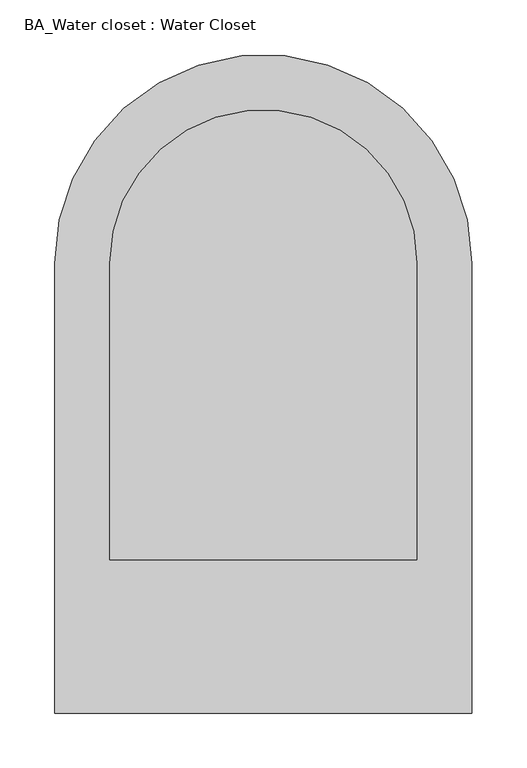
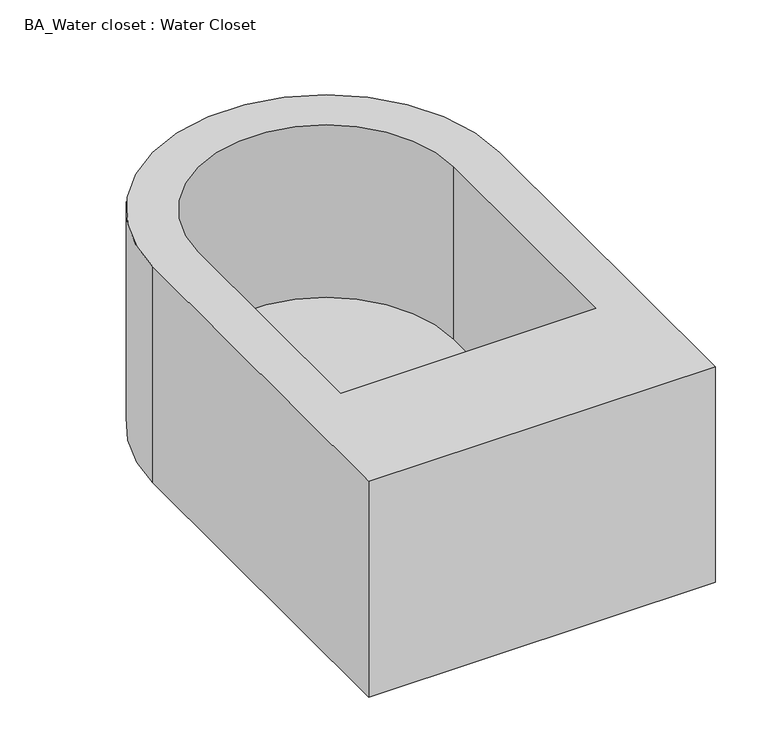
"""IFC4 building model written with IfcOpenShell, lengths in millimetres: flow terminal geometry, BA_Water closet : Water Closet."""

from ifc_helpers import new_model, si_unit, frame, origin, place, context, project, spatial, polyline, circle_curve, source, transform, mapped, element, save
from ifc_brep_helpers import plane_surface, cylinder_surface, revolved_surface, advanced_brep


def ba_water_closet_water_closet_d6486678(model_context):
    return source(origin(), model_context, "Body", "AdvancedBrep", [
        advanced_brep(
        [(-65.0, 560.0, 400.0), (-65.0, 150.0, 400.0), (315.0, 150.0, 400.0), (315.0, 560.0, 400.0), (-15.0, 290.0, 400.0), (-15.0, 560.0, 400.0), (265.0, 560.0, 400.0), (265.0, 290.0, 400.0), (-65.0, 560.0, 150.0), (315.0, 560.0, 150.0), (315.0, 150.0, 150.0), (-65.0, 150.0, 150.0), (-15.0, 560.0, 200.0), (-15.0, 290.0, 200.0), (265.0, 290.0, 200.0), (265.0, 560.0, 200.0)],
        [
            (0, 1),
            (1, 2),
            (2, 3),
            (3, 0, circle_curve(frame((125.0, 560.0, 400.0), z_axis=(0.0, 0.0, 1.0), x_axis=(-1.0, 0.0, 0.0)), 190.0)),
            (4, 5),
            (5, 6, circle_curve(frame((125.0, 560.0, 400.0), z_axis=(0.0, 0.0, -1.0), x_axis=(-1.0, 0.0, 0.0)), 140.0)),
            (6, 7),
            (7, 4),
            (8, 9, circle_curve(frame((125.0, 560.0, 150.0), z_axis=(0.0, 0.0, -1.0), x_axis=(-1.0, 0.0, 0.0)), 190.0)),
            (9, 10),
            (10, 11),
            (11, 8),
            (0, 8),
            (11, 1),
            (10, 2),
            (9, 3),
            (12, 13),
            (13, 14),
            (14, 15),
            (15, 12, circle_curve(frame((125.0, 560.0, 200.0), z_axis=(0.0, 0.0, 1.0), x_axis=(-1.0, 0.0, 0.0)), 140.0)),
            (12, 5),
            (4, 13),
            (7, 14),
            (6, 15),
        ],
        [
            plane_surface(frame((-65.0, 150.0, 400.0), z_axis=(0.0, 0.0, 1.0), x_axis=(0.0, -1.0, 0.0))),
            plane_surface(frame((-65.0, 150.0, 150.0), z_axis=(0.0, 0.0, -1.0), x_axis=(0.0, 1.0, 0.0))),
            plane_surface(frame((-65.0, 560.0, 400.0), z_axis=(-1.0, 0.0, 0.0), x_axis=(0.0, 0.0, -1.0))),
            plane_surface(frame((-65.0, 150.0, 400.0), z_axis=(0.0, -1.0, 0.0), x_axis=(0.0, 0.0, -1.0))),
            plane_surface(frame((315.0, 150.0, 400.0), z_axis=(1.0, 0.0, 0.0), x_axis=(0.0, 0.0, -1.0))),
            plane_surface(frame((-15.0, 290.0, 200.0), z_axis=(0.0, 0.0, 1.0), x_axis=(0.0, 1.0, 0.0))),
            plane_surface(frame((-15.0, 560.0, 400.0), z_axis=(1.0, 0.0, 0.0), x_axis=(0.0, 0.0, -1.0))),
            plane_surface(frame((-15.0, 290.0, 400.0), z_axis=(0.0, 1.0, 0.0), x_axis=(0.0, 0.0, -1.0))),
            plane_surface(frame((265.0, 290.0, 400.0), z_axis=(-1.0, 0.0, 0.0), x_axis=(0.0, 0.0, -1.0))),
            cylinder_surface(frame((125.0, 560.0, 150.0), z_axis=(0.0, 0.0, 1.0), x_axis=(-1.0, 0.0, 0.0)), 190.0),
            revolved_surface(polyline([(-15.0, 560.0, 400.0), (-15.0, 560.0, 200.0)]), (125.0, 560.0, 200.0), (0.0, 0.0, 1.0)),
        ],
        [
            (0, [[1, 2, 3, 4], [5, 6, 7, 8]]),
            (1, [[9, 10, 11, 12]]),
            (2, [[-1, 13, -12, 14]]),
            (3, [[-2, -14, -11, 15]]),
            (4, [[-3, -15, -10, 16]]),
            (5, [[17, 18, 19, 20]]),
            (6, [[-17, 21, -5, 22]]),
            (7, [[-18, -22, -8, 23]]),
            (8, [[-19, -23, -7, 24]]),
            (9, [[-4, -16, -9, -13]]),
            (10, [[-20, -24, -6, -21]]),
        ],
    ),
    ])


if __name__ == "__main__":
    model = new_model("IFC4")
    model_context = context("Model", 3, world=origin())
    ifc_project = project(units=[si_unit("LENGTHUNIT", "METRE", prefix="MILLI")], contexts=[model_context])
    site = spatial("IfcSite", under=ifc_project)
    building = spatial("IfcBuilding", under=site)
    placement = place(None, origin())
    ba_water_closet_water_closet_shape = ba_water_closet_water_closet_d6486678(model_context)
    element("IfcFlowTerminal", 1, ObjectType="BA_Water closet : Water Closet", at=placement, inside=building, context=model_context, shape_type="MappedRepresentation", body=[
        mapped(ba_water_closet_water_closet_shape, transform((0.0, 0.0, 0.0), x_axis=(1.0, 0.0, 0.0), y_axis=(0.0, 1.0, 0.0), z_axis=(0.0, 0.0, 1.0))),
    ])
    save(model, "model.ifc")

# Revit data of these elements
# Type "BA_Water closet : Water Closet"
#   height = 400 mm
#   width = 380 mm
#   depth = 600 mm
#   Default Elevation = 0
# Element 1 (IfcFlowTerminal, "BA_Water closet : Water Closet")
#   Materials on its faces: "Default"
# Materials
#   "Default": class "Generic", colour RGB 255 255 255, transparency 0, Cost = 0
